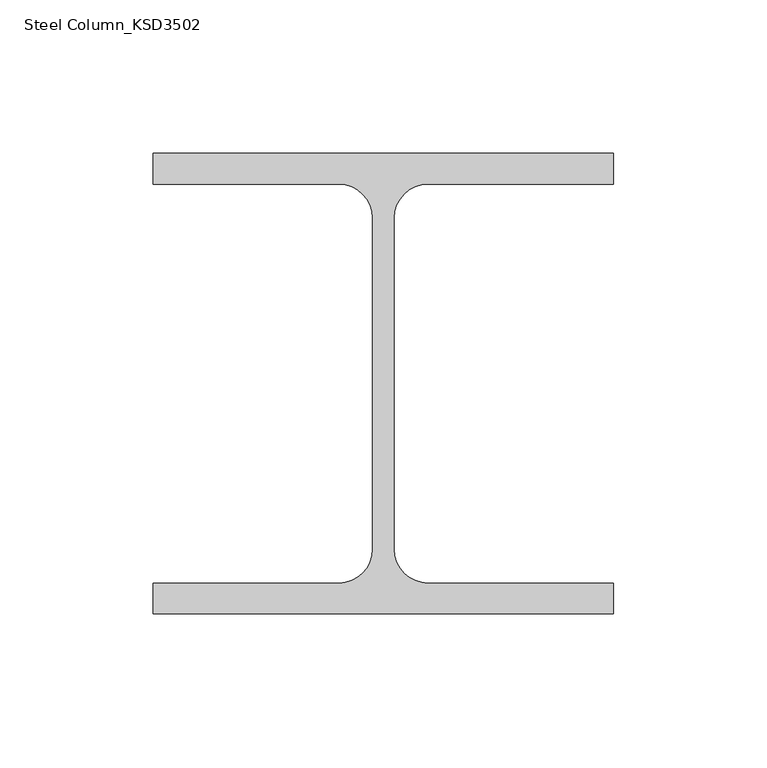
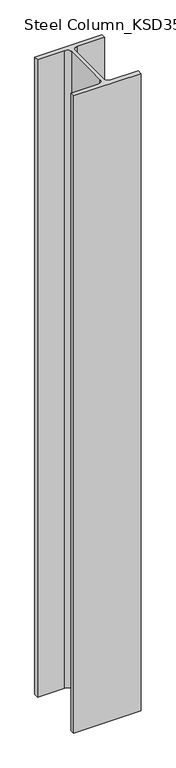
"""IFC4 building model written with IfcOpenShell, lengths in millimetres: column geometry, Steel Column_KSD3502 : H_SC_ASC_H-150×150x7x10."""

from ifc_helpers import new_model, si_unit, point, frame, frame_2d, origin, place, context, project, spatial, polyline, circle_curve, trimmed, segment, composite_curve, outline, extrude, source, transform, mapped, element, save


def steel_column_ksd3502_0d301b3b(model_context):
    return source(origin(), model_context, "Body", "SweptSolid", [
        extrude(outline(composite_curve([segment(polyline([(75.0, 75.0), (75.0, 65.0), (14.5, 65.0)]), True, "CONTINUOUS"), segment(trimmed(circle_curve(frame_2d((14.5, 54.0)), 11.0), [point((14.5, 65.0))], [point((3.5, 54.0))], True, "CARTESIAN"), True, "CONTINUOUS"), segment(polyline([(3.5, 54.0), (3.5, -54.0)]), True, "CONTINUOUS"), segment(trimmed(circle_curve(frame_2d((14.5, -54.0)), 11.0), [point((3.5, -54.0))], [point((14.5, -65.0))], True, "CARTESIAN"), True, "CONTINUOUS"), segment(polyline([(14.5, -65.0), (75.0, -65.0), (75.0, -75.0), (-75.0, -75.0), (-75.0, -65.0), (-14.5, -65.0)]), True, "CONTINUOUS"), segment(trimmed(circle_curve(frame_2d((-14.5, -54.0)), 11.0), [point((-14.5, -65.0))], [point((-3.5, -54.0))], True, "CARTESIAN"), True, "CONTINUOUS"), segment(polyline([(-3.5, -54.0), (-3.5, 54.0)]), True, "CONTINUOUS"), segment(trimmed(circle_curve(frame_2d((-14.5, 54.0)), 11.0), [point((-3.5, 54.0))], [point((-14.5, 65.0))], True, "CARTESIAN"), True, "CONTINUOUS"), segment(polyline([(-14.5, 65.0), (-75.0, 65.0), (-75.0, 75.0), (75.0, 75.0)]), True, "CONTINUOUS")], self_intersect=False)), frame((0.0, 0.0, 6299.9720055), z_axis=(0.0, 0.0, 1.0), x_axis=(1.0, 0.0, 0.0)), (0.0, 0.0, 1.0), 1500.0),
    ])


if __name__ == "__main__":
    model = new_model("IFC4")
    model_context = context("Model", 3, world=origin())
    ifc_project = project(units=[si_unit("LENGTHUNIT", "METRE", prefix="MILLI")], contexts=[model_context])
    site = spatial("IfcSite", under=ifc_project)
    building = spatial("IfcBuilding", under=site)
    placement = place(None, origin())
    steel_column_ksd3502_shape = steel_column_ksd3502_0d301b3b(model_context)
    element("IfcColumn", 1, ObjectType="Steel Column_KSD3502 : H_SC_ASC_H-150×150x7x10", at=placement, inside=building, context=model_context, shape_type="MappedRepresentation", body=[
        mapped(steel_column_ksd3502_shape, transform((0.0, 0.0, 0.0), x_axis=(1.0, 0.0, 0.0), y_axis=(0.0, 1.0, 0.0), z_axis=(0.0, 0.0, 1.0))),
    ])
    save(model, "model.ifc")

# Revit data of these elements
# Type "Steel Column_KSD3502 : H_SC_ASC_H-150×150x7x10"
#   Width = 15.0 cm
#   Web Thickness = 0.7 cm
#   Web Fillet = 1.1 cm
#   Warping Constant = 27562.5 cm⁶
#   Torsional Moment of Inertia = 11.6007 cm⁴
#   Section Area = 40.14 cm²
#   Plastic Modulus weak axis = 115.0 cm³
#   Plastic Modulus strong axis = 246.0 cm³
#   Perimeter = 1.27 m²/m
#   Nominal Weight = 31.50 kgf/m
#   Moment of Inertia weak axis = 563.00 cm⁴
#   Moment of Inertia strong axis = 1640.00 cm⁴
#   Height = 15.0 cm
#   Flange Thickness = 1.0 cm
#   Elastic Modulus weak axis = 75.1 cm³
#   Elastic Modulus strong axis = 219.0 cm³
#   Centroid Vertical = 7.5 cm
#   Centroid Horizontal = 7.5 cm
#   Bolt Spacing = 13.97 cm
#   Structural Material [instance default] = Steel, 45-345
#   Section Name Key = ""
#   Assembly Code = ""
# Element 1 (IfcColumn, "Steel Column_KSD3502 : H_SC_ASC_H-150×150x7x10")
#   Structural Material = none
# Materials
#   "Steel, 45-345": class "Metal", colour RGB 189 187 185, transparency 0, Description = "Steel 345 MPa", Cost = 0
